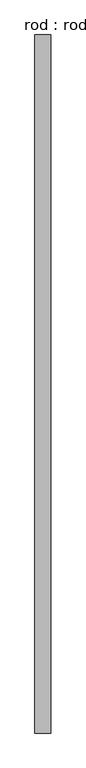
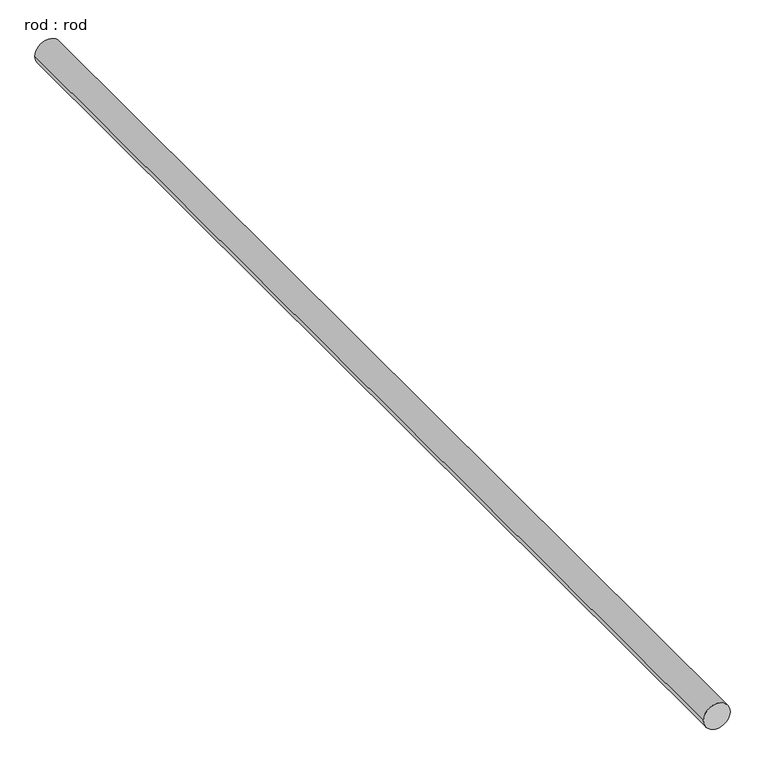
"""IFC4 building model written with IfcOpenShell, lengths in millimetres: proxy geometry, rod : rod."""

from ifc_helpers import new_model, si_unit, point, frame, frame_2d, origin, place, context, project, spatial, circle_curve, trimmed, segment, composite_curve, outline, extrude, source, transform, mapped, element, save


def rod_rod_dbdeafbe(model_context):
    return source(origin(), model_context, "Body", "SweptSolid", [
        extrude(outline(composite_curve([segment(trimmed(circle_curve(frame_2d((0.0108462, 0.0)), 200.0), [point((0.0108462, 200.0))], [point((0.0108462, -200.0))], False, "CARTESIAN"), True, "CONTINUOUS"), segment(trimmed(circle_curve(frame_2d((0.0108462, 0.0)), 200.0), [point((0.0108462, -200.0))], [point((0.0108462, 200.0))], False, "CARTESIAN"), True, "CONTINUOUS")], self_intersect=False)), frame((0.0, -4599.2356704, 0.0), z_axis=(0.0, 1.0, 0.0), x_axis=(0.0, 0.0, 1.0)), (0.0, 0.0, 1.0), 17383.9285714),
    ])


if __name__ == "__main__":
    model = new_model("IFC4")
    model_context = context("Model", 3, world=origin())
    ifc_project = project(units=[si_unit("LENGTHUNIT", "METRE", prefix="MILLI")], contexts=[model_context])
    site = spatial("IfcSite", under=ifc_project)
    building = spatial("IfcBuilding", under=site)
    placement = place(None, origin())
    rod_rod_shape = rod_rod_dbdeafbe(model_context)
    element("IfcBuildingElementProxy", 1, Name="rod : rod", ObjectType="rod : rod", at=placement, inside=building, context=model_context, shape_type="MappedRepresentation", body=[
        mapped(rod_rod_shape, transform((0.0, 0.0, 0.0), x_axis=(1.0, 0.0, 0.0), y_axis=(0.0, 1.0, 0.0), z_axis=(0.0, 0.0, 1.0))),
    ])
    save(model, "model.ifc")

# Revit data of these elements
# Type "rod : rod"
#   Default Elevation = 0
